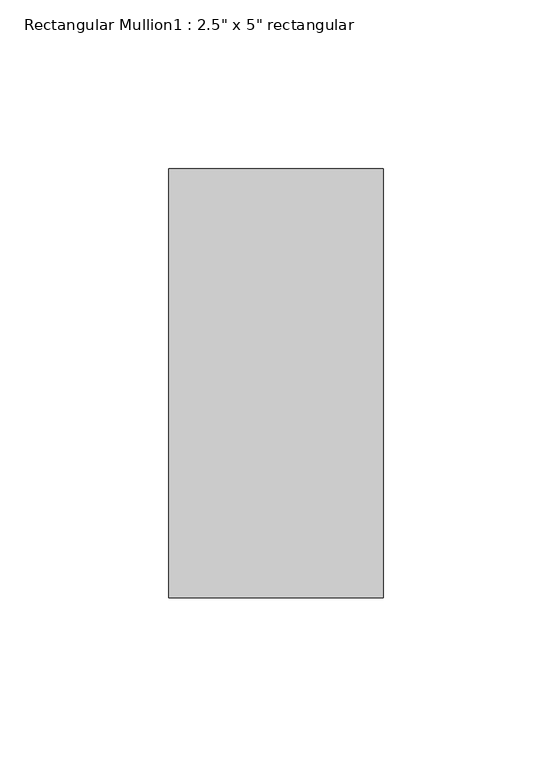
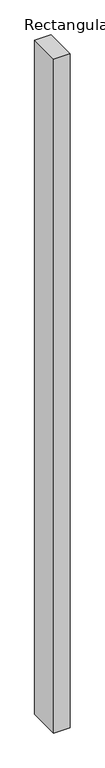
"""IFC4 building model written with IfcOpenShell, lengths in millimetres: member geometry."""

import ifcopenshell
import ifcopenshell.guid

model = None  # the IFC model being written
_history = None  # IfcOwnerHistory: only IFC2X3 demands one
_inside = {}  # id of a spatial element -> (the spatial element, [elements in it])
_under = {}  # id of a project, library or spatial element -> (it, [spatial elements below it])
_declared = {}  # id of a project -> (the project, [libraries it declares])
_typed = {}  # id of a type object -> (the type object, [elements of that type])
_made_of = {}  # id of a material, layer set ... -> (it, [elements and type objects made of it])


def new_model(schema):
    """Start an empty IFC model of exactly this schema.

    Asked for "IFC4X3", IfcOpenShell would pick the latest addendum, in which some entities
    have other attributes; the version numbers below select the first issue.
    IFC2X3 requires an IfcOwnerHistory on every rooted entity: one is made here for all.
    """
    global model, _history
    if schema == "IFC4X3":
        model = ifcopenshell.file(schema_version=(4, 3, 0, 0))
    else:
        model = ifcopenshell.file(schema=schema)
    _inside.clear()
    _under.clear()
    _declared.clear()
    _typed.clear()
    _made_of.clear()
    _history = None
    if model.schema == "IFC2X3":
        org = make("IfcOrganization", Name="unknown")
        user = make(
            "IfcPersonAndOrganization",
            ThePerson=make("IfcPerson", FamilyName="unknown"),
            TheOrganization=org,
        )
        app = make(
            "IfcApplication",
            ApplicationDeveloper=org,
            Version="unknown",
            ApplicationFullName="unknown",
            ApplicationIdentifier="unknown",
        )
        _history = make(
            "IfcOwnerHistory",
            OwningUser=user,
            OwningApplication=app,
            ChangeAction="ADDED",
            CreationDate=0,
        )
    return model


def make(cls, **values):
    """One entity of the class cls with the attributes given. An attribute that is None is left unset."""
    return model.create_entity(
        cls, **{name: value for name, value in values.items() if value is not None}
    )


def rooted(cls, **values):
    """An entity with a GlobalId (a new one), such as an element, a storey or a relation."""
    return make(cls, GlobalId=ifcopenshell.guid.new(), OwnerHistory=_history, **values)


def si_unit(unit_type, name, prefix=None):
    """IfcSIUnit, for example si_unit("LENGTHUNIT", "METRE", prefix="MILLI")."""
    return make("IfcSIUnit", UnitType=unit_type, Prefix=prefix, Name=name)


def assignment(units):
    """IfcUnitAssignment: the units of a project."""
    return None if units is None else make("IfcUnitAssignment", Units=units)


def point(xyz):
    """IfcCartesianPoint."""
    return None if xyz is None else make("IfcCartesianPoint", Coordinates=xyz)


def direction(xyz):
    """IfcDirection."""
    return None if xyz is None else make("IfcDirection", DirectionRatios=xyz)


def frame(location, z_axis=None, x_axis=None):
    """IfcAxis2Placement3D, a coordinate frame: its origin and axes. An axis left out is left unset."""
    return make(
        "IfcAxis2Placement3D",
        Location=point(location),
        Axis=direction(z_axis),
        RefDirection=direction(x_axis),
    )


def origin():
    """The frame at (0, 0, 0) with its axes left unset."""
    return frame((0.0, 0.0, 0.0))


def place(relative_to, where):
    """IfcLocalPlacement: puts the frame where relative to a parent placement (None: the world)."""
    return make(
        "IfcLocalPlacement", PlacementRelTo=relative_to, RelativePlacement=where
    )


def context(
    kind, dimensions, precision=None, world=None, true_north=None, identifier=None
):
    """IfcGeometricRepresentationContext, for example the 3D "Model" context."""
    return make(
        "IfcGeometricRepresentationContext",
        ContextIdentifier=identifier,
        ContextType=kind,
        CoordinateSpaceDimension=dimensions,
        Precision=precision,
        WorldCoordinateSystem=world,
        TrueNorth=true_north,
    )


def project(units=None, contexts=None):
    """IfcProject with its units and contexts."""
    return rooted(
        "IfcProject",
        Name="project",
        RepresentationContexts=contexts,
        UnitsInContext=assignment(units),
    )


def spatial(cls, under=None, at=None, **own):
    """A site, building, storey or space (cls), placed at a placement, below another one or the project."""
    s = rooted(cls, ObjectPlacement=at, **own)
    if under is not None:
        _under.setdefault(under.id(), (under, []))[1].append(s)
    return s


def polyline(points):
    """IfcPolyline through the points."""
    return make("IfcPolyline", Points=[point(p) for p in points])


def outline(outer, holes=None, kind="AREA"):
    """IfcArbitraryClosedProfileDef: a profile drawn as a closed curve; with holes, ...WithVoids."""
    if holes is None:
        return make("IfcArbitraryClosedProfileDef", ProfileType=kind, OuterCurve=outer)
    return make(
        "IfcArbitraryProfileDefWithVoids",
        ProfileType=kind,
        OuterCurve=outer,
        InnerCurves=holes,
    )


def extrude(swept, where, along, depth):
    """IfcExtrudedAreaSolid: the profile swept, set in the frame where, extruded along a direction by depth."""
    return make(
        "IfcExtrudedAreaSolid",
        SweptArea=swept,
        Position=where,
        ExtrudedDirection=direction(along),
        Depth=depth,
    )


def shape(context_of_items, identifier, shape_type, items):
    """IfcShapeRepresentation: the items that make up one representation, for example the "Body"."""
    return make(
        "IfcShapeRepresentation",
        ContextOfItems=context_of_items,
        RepresentationIdentifier=identifier,
        RepresentationType=shape_type,
        Items=items,
    )


def source(mapping_origin, context_of_items, identifier, shape_type, items):
    """IfcRepresentationMap: a shape defined once, which mapped items show again and again."""
    return make(
        "IfcRepresentationMap",
        MappingOrigin=mapping_origin,
        MappedRepresentation=shape(context_of_items, identifier, shape_type, items),
    )


def transform(
    local_origin,
    x_axis=None,
    y_axis=None,
    z_axis=None,
    scale=None,
    scale2=None,
    scale3=None,
    uniform=True,
):
    """IfcCartesianTransformationOperator3D, or its non-uniform kind. x_axis, y_axis, z_axis: its Axis1, 2, 3."""
    if uniform:
        return make(
            "IfcCartesianTransformationOperator3D",
            Axis1=direction(x_axis),
            Axis2=direction(y_axis),
            LocalOrigin=point(local_origin),
            Scale=scale,
            Axis3=direction(z_axis),
        )
    return make(
        "IfcCartesianTransformationOperator3DnonUniform",
        Axis1=direction(x_axis),
        Axis2=direction(y_axis),
        LocalOrigin=point(local_origin),
        Scale=scale,
        Axis3=direction(z_axis),
        Scale2=scale2,
        Scale3=scale3,
    )


def mapped(mapping_source, mapping_target):
    """IfcMappedItem: shows the shape of a source again, moved by a transform."""
    return make(
        "IfcMappedItem", MappingSource=mapping_source, MappingTarget=mapping_target
    )


def made_of(thing, what):
    """Note that an element or type object is made of a material, layer set ...; save() writes the relation."""
    if what is not None:
        _made_of.setdefault(what.id(), (what, []))[1].append(thing)
    return thing


def element(
    cls,
    number,
    at=None,
    inside=None,
    cuts=None,
    type_object=None,
    material=None,
    context=None,
    identifier="Body",
    shape_type=None,
    held_by="IfcProductDefinitionShape",
    body=None,
    shapes=None,
    **own,
):
    """One element of the class cls, such as IfcWall. Its Tag is "e" and its number.

    at: its placement. inside: the storey or other place that contains it. cuts: it is an
    opening in that element (IfcRelVoidsElement). A single representation is given by context,
    identifier, shape_type and body (its items); several are given by shapes. held_by: the class
    of the entity that holds the representations. save() writes the other relations.
    """
    e = rooted(cls, Tag="e%d" % number, ObjectPlacement=at, **own)
    if body is not None:
        shapes = [shape(context, identifier, shape_type, body)]
    if shapes is not None:
        e.Representation = make(held_by, Representations=shapes)
    if inside is not None:
        _inside.setdefault(inside.id(), (inside, []))[1].append(e)
    if cuts is not None:
        rooted(
            "IfcRelVoidsElement", RelatingBuildingElement=cuts, RelatedOpeningElement=e
        )
    if type_object is not None:
        _typed.setdefault(type_object.id(), (type_object, []))[1].append(e)
    return made_of(e, material)


def aggregate(whole, parts):
    """IfcRelAggregates: a whole, such as a stair, and the parts it consists of."""
    return rooted("IfcRelAggregates", RelatingObject=whole, RelatedObjects=parts)


def save(model, path):
    """Write the relations noted so far, then the file.

    IfcRelAggregates (storeys below a building ...), IfcRelContainedInSpatialStructure (elements
    in a storey), IfcRelDefinesByType, IfcRelAssociatesMaterial and IfcRelDeclares: one each for
    every whole, place, type object, material and project.
    """
    for whole, parts in _under.values():
        aggregate(whole, parts)
    for where, things in _inside.values():
        rooted(
            "IfcRelContainedInSpatialStructure",
            RelatedElements=things,
            RelatingStructure=where,
        )
    for kind, things in _typed.values():
        rooted("IfcRelDefinesByType", RelatedObjects=things, RelatingType=kind)
    for what, things in _made_of.values():
        rooted("IfcRelAssociatesMaterial", RelatedObjects=things, RelatingMaterial=what)
    for by, libraries in _declared.values():
        rooted("IfcRelDeclares", RelatingContext=by, RelatedDefinitions=libraries)
    model.write(path)


def member_923d5781(model_context):
    return source(origin(), model_context, "Body", "SweptSolid", [
        extrude(outline(polyline([(31.75, 63.5), (31.75, -63.5), (-31.75, -63.5), (-31.75, 63.5), (31.75, 63.5)])), frame((0.0, 0.0, -2743.2), z_axis=(0.0, 0.0, 1.0), x_axis=(1.0, 0.0, 0.0)), (0.0, 0.0, 1.0), 2743.2),
    ])


if __name__ == "__main__":
    model = new_model("IFC4")
    model_context = context("Model", 3, world=origin())
    ifc_project = project(units=[si_unit("LENGTHUNIT", "METRE", prefix="MILLI")], contexts=[model_context])
    site = spatial("IfcSite", under=ifc_project)
    building = spatial("IfcBuilding", under=site)
    placement = place(None, origin())
    member_shape = member_923d5781(model_context)
    element("IfcMember", 1, ObjectType="Rectangular Mullion1 : 2.5\" x 5\" rectangular", at=placement, inside=building, context=model_context, shape_type="MappedRepresentation", body=[
        mapped(member_shape, transform((0.0, 0.0, 0.0), x_axis=(1.0, 0.0, 0.0), y_axis=(0.0, 1.0, 0.0), z_axis=(0.0, 0.0, 1.0))),
    ])
    save(model, "model.ifc")

# Revit data of these elements
# Type "Rectangular Mullion1 : 2.5\" x 5\" rectangular"
#   built-in parameter 1007304 = 0.416667 (stored number, unit not read)
#   built-in parameter 1007301 = 0.104167 (stored number, unit not read)
#   built-in parameter 1007300 = 0.104167 (stored number, unit not read)
# Element 1 (IfcMember, "Rectangular Mullion1 : 2.5\" x 5\" rectangular")
#   Materials on its faces: "support-frame"
# Materials
#   "support-frame": class "Unassigned", colour RGB 233 233 233, transparency 0, Cost = 0
